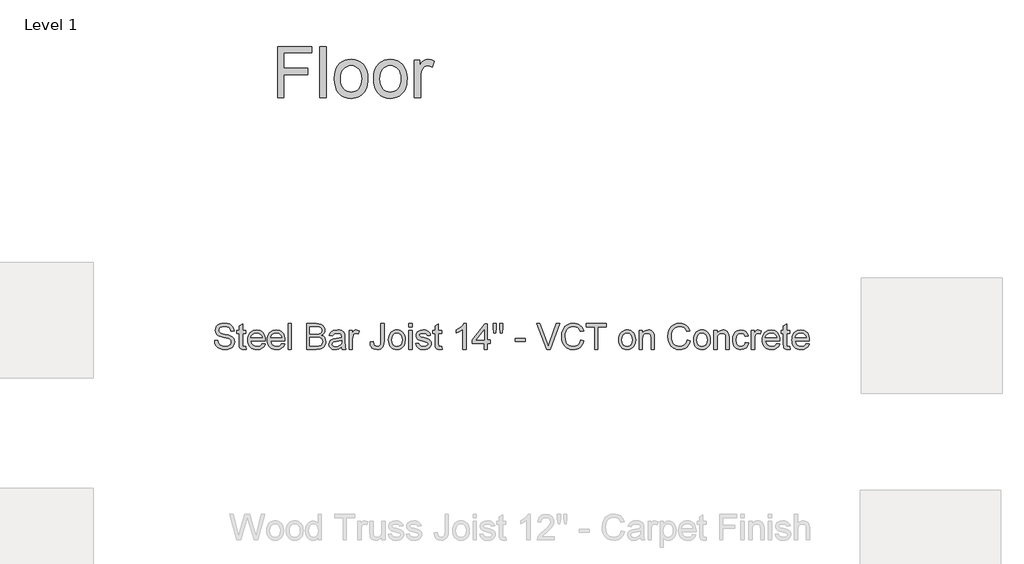
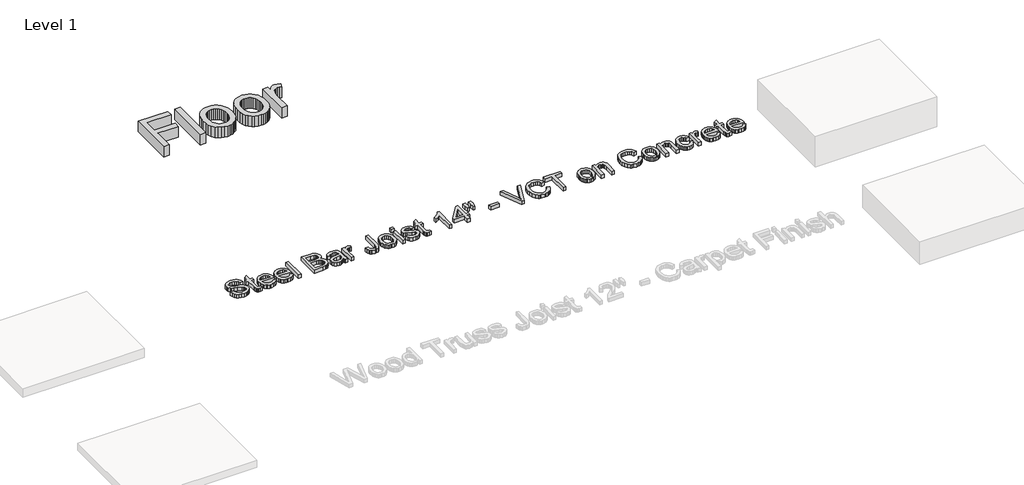
# One storey, part 18 of 42: 2 proxies.
"""IFC4 building model written with IfcOpenShell, lengths in millimetres."""

import ifcopenshell
import ifcopenshell.guid

model = None  # the IFC model being written
_history = None  # IfcOwnerHistory: only IFC2X3 demands one
_inside = {}  # id of a spatial element -> (the spatial element, [elements in it])
_under = {}  # id of a project, library or spatial element -> (it, [spatial elements below it])
_declared = {}  # id of a project -> (the project, [libraries it declares])
_typed = {}  # id of a type object -> (the type object, [elements of that type])
_made_of = {}  # id of a material, layer set ... -> (it, [elements and type objects made of it])


def new_model(schema):
    """Start an empty IFC model of exactly this schema.

    Asked for "IFC4X3", IfcOpenShell would pick the latest addendum, in which some entities
    have other attributes; the version numbers below select the first issue.
    IFC2X3 requires an IfcOwnerHistory on every rooted entity: one is made here for all.
    """
    global model, _history
    if schema == "IFC4X3":
        model = ifcopenshell.file(schema_version=(4, 3, 0, 0))
    else:
        model = ifcopenshell.file(schema=schema)
    _inside.clear()
    _under.clear()
    _declared.clear()
    _typed.clear()
    _made_of.clear()
    _history = None
    if model.schema == "IFC2X3":
        org = make("IfcOrganization", Name="unknown")
        user = make(
            "IfcPersonAndOrganization",
            ThePerson=make("IfcPerson", FamilyName="unknown"),
            TheOrganization=org,
        )
        app = make(
            "IfcApplication",
            ApplicationDeveloper=org,
            Version="unknown",
            ApplicationFullName="unknown",
            ApplicationIdentifier="unknown",
        )
        _history = make(
            "IfcOwnerHistory",
            OwningUser=user,
            OwningApplication=app,
            ChangeAction="ADDED",
            CreationDate=0,
        )
    return model


def make(cls, **values):
    """One entity of the class cls with the attributes given. An attribute that is None is left unset."""
    return model.create_entity(
        cls, **{name: value for name, value in values.items() if value is not None}
    )


def rooted(cls, **values):
    """An entity with a GlobalId (a new one), such as an element, a storey or a relation."""
    return make(cls, GlobalId=ifcopenshell.guid.new(), OwnerHistory=_history, **values)


def si_unit(unit_type, name, prefix=None):
    """IfcSIUnit, for example si_unit("LENGTHUNIT", "METRE", prefix="MILLI")."""
    return make("IfcSIUnit", UnitType=unit_type, Prefix=prefix, Name=name)


def assignment(units):
    """IfcUnitAssignment: the units of a project."""
    return None if units is None else make("IfcUnitAssignment", Units=units)


def point(xyz):
    """IfcCartesianPoint."""
    return None if xyz is None else make("IfcCartesianPoint", Coordinates=xyz)


def direction(xyz):
    """IfcDirection."""
    return None if xyz is None else make("IfcDirection", DirectionRatios=xyz)


def frame(location, z_axis=None, x_axis=None):
    """IfcAxis2Placement3D, a coordinate frame: its origin and axes. An axis left out is left unset."""
    return make(
        "IfcAxis2Placement3D",
        Location=point(location),
        Axis=direction(z_axis),
        RefDirection=direction(x_axis),
    )


def origin():
    """The frame at (0, 0, 0) with its axes left unset."""
    return frame((0.0, 0.0, 0.0))


def origin_with_axes():
    """The frame at (0, 0, 0) with the z axis (0, 0, 1) and the x axis (1, 0, 0) written out."""
    return frame((0.0, 0.0, 0.0), z_axis=(0.0, 0.0, 1.0), x_axis=(1.0, 0.0, 0.0))


def place(relative_to, where):
    """IfcLocalPlacement: puts the frame where relative to a parent placement (None: the world)."""
    return make(
        "IfcLocalPlacement", PlacementRelTo=relative_to, RelativePlacement=where
    )


def context(
    kind, dimensions, precision=None, world=None, true_north=None, identifier=None
):
    """IfcGeometricRepresentationContext, for example the 3D "Model" context."""
    return make(
        "IfcGeometricRepresentationContext",
        ContextIdentifier=identifier,
        ContextType=kind,
        CoordinateSpaceDimension=dimensions,
        Precision=precision,
        WorldCoordinateSystem=world,
        TrueNorth=true_north,
    )


def project(units=None, contexts=None):
    """IfcProject with its units and contexts."""
    return rooted(
        "IfcProject",
        Name="project",
        RepresentationContexts=contexts,
        UnitsInContext=assignment(units),
    )


def spatial(cls, under=None, at=None, **own):
    """A site, building, storey or space (cls), placed at a placement, below another one or the project."""
    s = rooted(cls, ObjectPlacement=at, **own)
    if under is not None:
        _under.setdefault(under.id(), (under, []))[1].append(s)
    return s


def polyline(points):
    """IfcPolyline through the points."""
    return make("IfcPolyline", Points=[point(p) for p in points])


def outline(outer, holes=None, kind="AREA"):
    """IfcArbitraryClosedProfileDef: a profile drawn as a closed curve; with holes, ...WithVoids."""
    if holes is None:
        return make("IfcArbitraryClosedProfileDef", ProfileType=kind, OuterCurve=outer)
    return make(
        "IfcArbitraryProfileDefWithVoids",
        ProfileType=kind,
        OuterCurve=outer,
        InnerCurves=holes,
    )


def extrude(swept, where, along, depth):
    """IfcExtrudedAreaSolid: the profile swept, set in the frame where, extruded along a direction by depth."""
    return make(
        "IfcExtrudedAreaSolid",
        SweptArea=swept,
        Position=where,
        ExtrudedDirection=direction(along),
        Depth=depth,
    )


def shape(context_of_items, identifier, shape_type, items):
    """IfcShapeRepresentation: the items that make up one representation, for example the "Body"."""
    return make(
        "IfcShapeRepresentation",
        ContextOfItems=context_of_items,
        RepresentationIdentifier=identifier,
        RepresentationType=shape_type,
        Items=items,
    )


def made_of(thing, what):
    """Note that an element or type object is made of a material, layer set ...; save() writes the relation."""
    if what is not None:
        _made_of.setdefault(what.id(), (what, []))[1].append(thing)
    return thing


def element(
    cls,
    number,
    at=None,
    inside=None,
    cuts=None,
    type_object=None,
    material=None,
    context=None,
    identifier="Body",
    shape_type=None,
    held_by="IfcProductDefinitionShape",
    body=None,
    shapes=None,
    **own,
):
    """One element of the class cls, such as IfcWall. Its Tag is "e" and its number.

    at: its placement. inside: the storey or other place that contains it. cuts: it is an
    opening in that element (IfcRelVoidsElement). A single representation is given by context,
    identifier, shape_type and body (its items); several are given by shapes. held_by: the class
    of the entity that holds the representations. save() writes the other relations.
    """
    e = rooted(cls, Tag="e%d" % number, ObjectPlacement=at, **own)
    if body is not None:
        shapes = [shape(context, identifier, shape_type, body)]
    if shapes is not None:
        e.Representation = make(held_by, Representations=shapes)
    if inside is not None:
        _inside.setdefault(inside.id(), (inside, []))[1].append(e)
    if cuts is not None:
        rooted(
            "IfcRelVoidsElement", RelatingBuildingElement=cuts, RelatedOpeningElement=e
        )
    if type_object is not None:
        _typed.setdefault(type_object.id(), (type_object, []))[1].append(e)
    return made_of(e, material)


def aggregate(whole, parts):
    """IfcRelAggregates: a whole, such as a stair, and the parts it consists of."""
    return rooted("IfcRelAggregates", RelatingObject=whole, RelatedObjects=parts)


def save(model, path):
    """Write the relations noted so far, then the file.

    IfcRelAggregates (storeys below a building ...), IfcRelContainedInSpatialStructure (elements
    in a storey), IfcRelDefinesByType, IfcRelAssociatesMaterial and IfcRelDeclares: one each for
    every whole, place, type object, material and project.
    """
    for whole, parts in _under.values():
        aggregate(whole, parts)
    for where, things in _inside.values():
        rooted(
            "IfcRelContainedInSpatialStructure",
            RelatedElements=things,
            RelatingStructure=where,
        )
    for kind, things in _typed.values():
        rooted("IfcRelDefinesByType", RelatedObjects=things, RelatingType=kind)
    for what, things in _made_of.values():
        rooted("IfcRelAssociatesMaterial", RelatedObjects=things, RelatingMaterial=what)
    for by, libraries in _declared.values():
        rooted("IfcRelDeclares", RelatingContext=by, RelatedDefinitions=libraries)
    model.write(path)


model = new_model("IFC4")

# Units and contexts
model_context = context("Model", 3, world=origin())
ifc_project = project(units=[si_unit("LENGTHUNIT", "METRE", prefix="MILLI")], contexts=[model_context])

# Site, building, storey
site = spatial("IfcSite", under=ifc_project)
building = spatial("IfcBuilding", under=site)
storey = spatial("IfcBuildingStorey", under=building, Name="Level 1", Elevation=0.0)

# Proxies
placement = place(None, origin())
element("IfcBuildingElementProxy", 1, Name="24\" Arial", ObjectType="24\" Arial", at=placement, inside=storey, context=model_context, shape_type="SweptSolid", body=[
    extrude(outline(polyline([(27657.5158557, -3283.876067), (27657.5158557, -2674.7418789), (28066.7778883, -2674.7418789), (28066.7778883, -2750.8836524), (27733.6576292, -2750.8836524), (27733.6576292, -2931.7203645), (28019.1892799, -2931.7203645), (28019.1892799, -3007.862138), (27733.6576292, -3007.862138), (27733.6576292, -3283.876067), (27657.5158557, -3283.876067)])), origin_with_axes(), (0.0, 0.0, 1.0), 152.4),
    extrude(outline(polyline([(28161.9551052, -3283.876067), (28161.9551052, -2674.7418789), (28238.0968788, -2674.7418789), (28238.0968788, -3283.876067), (28161.9551052, -3283.876067)])), origin_with_axes(), (0.0, 0.0, 1.0), 152.4),
    extrude(outline(polyline([(28333.2740956, -3060.2096073), (28337.3916256, -3002.2760533), (28349.7442156, -2952.3544877), (28370.3318655, -2910.4449104), (28399.1545755, -2876.5473216), (28428.172473, -2854.8814922), (28460.2018372, -2839.4058998), (28495.2426681, -2830.1205444), (28533.2949655, -2827.0254259), (28575.3021366, -2830.7944065), (28613.2847242, -2842.1013483), (28647.2427283, -2860.9462514), (28677.1761489, -2887.3291157), (28701.6071366, -2920.3576548), (28719.0578422, -2959.1395822), (28729.5282655, -3003.6748981), (28733.0184066, -3053.9636024), (28731.4754947, -3094.7206431), (28726.846759, -3130.8861266), (28719.1321994, -3162.4600529), (28708.331816, -3189.4424221), (28694.5803812, -3212.7487572), (28678.0126674, -3233.2945812), (28658.6286746, -3251.0798942), (28636.4284029, -3266.104696), (28612.2762547, -3278.0436741), (28587.0366323, -3286.5715155), (28560.709536, -3291.6882204), (28533.2949655, -3293.3937887), (28490.6743476, -3289.6387501), (28452.3385633, -3278.3736341), (28418.2876127, -3259.598441), (28388.5214958, -3233.3131705), (28364.3507582, -3199.963966), (28347.0859457, -3159.9969706), (28336.7270582, -3113.4121844), (28333.2740956, -3060.2096073)]), holes=[polyline([(28409.4158692, -3060.0608929), (28411.6187012, -3096.993185), (28418.2271974, -3128.9714286), (28429.2413578, -3155.9956238), (28444.6611823, -3178.0657704), (28463.4177862, -3195.2097525), (28484.4422847, -3207.455454), (28507.7346778, -3214.8028749), (28533.2949655, -3217.2520152), (28558.7251282, -3214.7889329), (28581.9245748, -3207.3996861), (28602.8933054, -3195.0842747), (28621.63132, -3177.8426988), (28637.0511445, -3155.5541279), (28648.0653048, -3128.0977315), (28654.673801, -3095.4735097), (28656.8766331, -3057.6814625), (28654.659859, -3021.9202963), (28648.0095369, -2990.7785711), (28636.9256667, -2964.2562871), (28621.4082484, -2942.3534442), (28602.6005239, -2925.2094621), (28581.6457353, -2912.9637606), (28558.5438825, -2905.6163397), (28533.2949655, -2903.1671994), (28507.7346778, -2905.6070451), (28484.4422847, -2912.926582), (28463.4177862, -2925.1258102), (28444.6611823, -2942.2047298), (28429.2413578, -2964.2098139), (28418.2271974, -2991.1875357), (28411.6187012, -3023.1378954), (28409.4158692, -3060.0608929)])]), origin_with_axes(), (0.0, 0.0, 1.0), 152.4),
    extrude(outline(polyline([(28799.6424584, -3060.2096073), (28803.7599884, -3002.2760533), (28816.1125784, -2952.3544877), (28836.7002283, -2910.4449104), (28865.5229383, -2876.5473216), (28894.5408358, -2854.8814922), (28926.5702, -2839.4058998), (28961.6110309, -2830.1205444), (28999.6633283, -2827.0254259), (29041.6704994, -2830.7944065), (29079.653087, -2842.1013483), (29113.6110911, -2860.9462514), (29143.5445117, -2887.3291157), (29167.9754994, -2920.3576548), (29185.426205, -2959.1395822), (29195.8966283, -3003.6748981), (29199.3867694, -3053.9636024), (29197.8438575, -3094.7206431), (29193.2151217, -3130.8861266), (29185.5005622, -3162.4600529), (29174.7001788, -3189.4424221), (29160.948744, -3212.7487572), (29144.3810302, -3233.2945812), (29124.9970374, -3251.0798942), (29102.7967657, -3266.104696), (29078.6446174, -3278.0436741), (29053.4049951, -3286.5715155), (29027.0778988, -3291.6882204), (28999.6633283, -3293.3937887), (28957.0427103, -3289.6387501), (28918.7069261, -3278.3736341), (28884.6559755, -3259.598441), (28854.8898586, -3233.3131705), (28830.719121, -3199.963966), (28813.4543085, -3159.9969706), (28803.0954209, -3113.4121844), (28799.6424584, -3060.2096073)]), holes=[polyline([(28875.784232, -3060.0608929), (28877.987064, -3096.993185), (28884.5955602, -3128.9714286), (28895.6097206, -3155.9956238), (28911.0295451, -3178.0657704), (28929.786149, -3195.2097525), (28950.8106475, -3207.455454), (28974.1030406, -3214.8028749), (28999.6633283, -3217.2520152), (29025.093491, -3214.7889329), (29048.2929376, -3207.3996861), (29069.2616682, -3195.0842747), (29087.9996828, -3177.8426988), (29103.4195073, -3155.5541279), (29114.4336676, -3128.0977315), (29121.0421638, -3095.4735097), (29123.2449959, -3057.6814625), (29121.0282218, -3021.9202963), (29114.3778997, -2990.7785711), (29103.2940295, -2964.2562871), (29087.7766112, -2942.3534442), (29068.9688867, -2925.2094621), (29048.0140981, -2912.9637606), (29024.9122453, -2905.6163397), (28999.6633283, -2903.1671994), (28974.1030406, -2905.6070451), (28950.8106475, -2912.926582), (28929.786149, -2925.1258102), (28911.0295451, -2942.2047298), (28895.6097206, -2964.2098139), (28884.5955602, -2991.1875357), (28877.987064, -3023.1378954), (28875.784232, -3060.0608929)])]), origin_with_axes(), (0.0, 0.0, 1.0), 152.4),
    extrude(outline(polyline([(29285.0462646, -3283.876067), (29285.0462646, -2836.5431476), (29351.6703164, -2836.5431476), (29351.6703164, -2902.7210562), (29376.2825499, -2864.3527407), (29398.9614961, -2841.7481516), (29421.7147995, -2830.7061073), (29446.5501045, -2827.0254259), (29484.4722769, -2832.8996448), (29522.9893069, -2850.5223013), (29497.5591442, -2918.7822116), (29470.790552, -2907.0709525), (29444.0219597, -2903.1671994), (29421.2872456, -2906.9222381), (29400.9691405, -2918.187354), (29384.5547884, -2936.1074393), (29373.5313334, -2959.8273863), (29364.273862, -3002.3597052), (29361.1880381, -3048.7585984), (29361.1880381, -3283.876067), (29285.0462646, -3283.876067)])), origin_with_axes(), (0.0, 0.0, 1.0), 152.4),
])
element("IfcBuildingElementProxy", 2, Name="8\" Arial", ObjectType="8\" Arial", at=placement, inside=storey, context=model_context, shape_type="SweptSolid", body=[
    extrude(outline(polyline([(26907.3095997, -6176.6357974), (26945.3804865, -6176.6357974), (26949.748972, -6197.762537), (26957.6494246, -6214.7438627), (26969.9741306, -6228.2211054), (26987.6153765, -6238.8355958), (27009.1789647, -6245.7229315), (27033.2706977, -6248.0187101), (27054.4810892, -6246.2806105), (27073.0518001, -6241.0663118), (27088.0998386, -6232.8126625), (27098.7422129, -6221.9565112), (27105.0718697, -6209.4923855), (27107.1817552, -6196.4148128), (27105.6016647, -6183.6718475), (27100.8613932, -6172.6576872), (27091.2321357, -6163.2607959), (27074.9850873, -6155.369638), (27019.5517942, -6140.8328053), (26983.1632391, -6131.2128424), (26959.8801406, -6122.0576121), (26940.9283491, -6109.2495843), (26927.4975797, -6093.7275186), (26919.494886, -6075.8260225), (26916.8273214, -6055.8797035), (26920.1269222, -6033.5818379), (26930.0257246, -6012.7897056), (26946.2634783, -5995.1670491), (26968.5799331, -5982.3776106), (26995.3671147, -5974.5979884), (27025.0170484, -5972.0047811), (27057.1393591, -5974.7188189), (27085.246381, -5982.8609324), (27108.3342918, -5996.2638178), (27125.3992694, -6014.7601715), (27136.1996528, -6037.1974568), (27140.4937811, -6062.4231371), (27102.4228944, -6062.4231371), (27095.4333175, -6039.7070123), (27080.8593062, -6023.3112495), (27058.0874135, -6013.3845633), (27026.5041925, -6010.0756678), (26994.1773995, -6013.3473847), (26972.0003643, -6023.1625351), (26959.1737472, -6037.6064214), (26954.8982082, -6054.7643454), (26957.9282641, -6069.3941247), (26967.0184319, -6081.1611517), (26988.5076629, -6091.6826956), (27029.1810517, -6102.4273111), (27071.1556915, -6112.6328369), (27096.5486755, -6121.5371117), (27118.2516835, -6135.3489617), (27133.3926685, -6152.39535), (27142.2876486, -6172.4903835), (27145.252642, -6195.4481692), (27141.8415054, -6218.9171606), (27131.6080957, -6240.9919546), (27114.970672, -6259.9902194), (27092.3474937, -6274.2296233), (27065.1420529, -6283.1246034), (27034.7578417, -6286.0895968), (26997.4584109, -6282.8922372), (26966.7581817, -6273.3001583), (26942.3039573, -6257.2761816), (26923.7425411, -6234.7831283), (26911.8267997, -6207.3824999), (26907.3095997, -6176.6357974)])), origin_with_axes(), (0.0, 0.0, 1.0), 50.8),
    extrude(outline(polyline([(27278.5007456, -6249.5802113), (27283.2596065, -6282.446094), (27254.7807986, -6286.0895968), (27236.5075165, -6284.5095063), (27222.8815595, -6279.7692348), (27213.252302, -6272.4636398), (27206.9691186, -6263.187579), (27203.5115087, -6247.2565488), (27202.3589721, -6219.9860454), (27202.3589721, -6095.735163), (27173.805807, -6095.735163), (27173.805807, -6057.6642763), (27202.3589721, -6057.6642763), (27202.3589721, -6003.3091626), (27240.4298589, -5980.9276451), (27240.4298589, -6057.6642763), (27278.5007456, -6057.6642763), (27278.5007456, -6095.735163), (27240.4298589, -6095.735163), (27240.4298589, -6218.8706874), (27242.4375033, -6238.5009884), (27248.9437584, -6245.4533866), (27261.9190899, -6248.0187101), (27278.5007456, -6249.5802113)])), origin_with_axes(), (0.0, 0.0, 1.0), 50.8),
    extrude(outline(polyline([(27473.1678971, -6214.7066841), (27510.4952118, -6219.465545), (27497.0458531, -6247.5911562), (27475.5845061, -6268.6156547), (27446.5944925, -6281.7211113), (27410.5591341, -6286.0895968), (27386.9367809, -6284.2051065), (27365.8890458, -6278.5516356), (27347.4159287, -6269.1291841), (27331.5174297, -6255.9377519), (27318.7326385, -6239.3444779), (27309.6006448, -6219.7165005), (27304.1214486, -6197.05382), (27302.2950499, -6171.3564361), (27304.1400379, -6144.7876789), (27309.675002, -6121.369808), (27318.8999422, -6101.1028235), (27331.8148585, -6083.9867253), (27347.6715316, -6070.3886522), (27365.7217421, -6060.6757429), (27385.9654899, -6054.8479973), (27408.4027753, -6052.9054154), (27430.1174015, -6054.84335), (27449.7546735, -6060.6571536), (27467.3145912, -6070.3468263), (27482.7971546, -6083.9123681), (27495.435555, -6100.9912877), (27504.4629839, -6121.2210936), (27509.8794413, -6144.6017859), (27511.684927, -6171.1333645), (27511.4618554, -6181.3946582), (27340.3659366, -6181.3946582), (27346.9558435, -6209.8920554), (27362.2641322, -6230.8421967), (27384.3575155, -6243.7245817), (27411.3027061, -6248.0187101), (27431.5650433, -6246.0296549), (27448.6300208, -6240.0624896), (27462.4976388, -6229.745428), (27473.1678971, -6214.7066841)]), holes=[polyline([(27340.3659366, -6143.3237715), (27473.6140403, -6143.3237715), (27468.4648041, -6123.2101487), (27458.3708141, -6108.8220304), (27436.1751897, -6095.4377342), (27408.2540609, -6090.9763022), (27382.591532, -6094.5361532), (27361.3718458, -6105.2157061), (27346.6212361, -6121.8624244), (27340.3659366, -6143.3237715)])]), origin_with_axes(), (0.0, 0.0, 1.0), 50.8),
    extrude(outline(polyline([(27706.3520785, -6214.7066841), (27743.6793932, -6219.465545), (27730.2300345, -6247.5911562), (27708.7686875, -6268.6156547), (27679.7786739, -6281.7211113), (27643.7433155, -6286.0895968), (27620.1209623, -6284.2051065), (27599.0732272, -6278.5516356), (27580.6001101, -6269.1291841), (27564.7016111, -6255.9377519), (27551.9168199, -6239.3444779), (27542.7848262, -6219.7165005), (27537.30563, -6197.05382), (27535.4792313, -6171.3564361), (27537.3242193, -6144.7876789), (27542.8591834, -6121.369808), (27552.0841236, -6101.1028235), (27564.9990399, -6083.9867253), (27580.855713, -6070.3886522), (27598.9059235, -6060.6757429), (27619.1496713, -6054.8479973), (27641.5869567, -6052.9054154), (27663.3015829, -6054.84335), (27682.9388549, -6060.6571536), (27700.4987726, -6070.3468263), (27715.981336, -6083.9123681), (27728.6197364, -6100.9912877), (27737.6471653, -6121.2210936), (27743.0636226, -6144.6017859), (27744.8691084, -6171.1333645), (27744.6460368, -6181.3946582), (27573.550118, -6181.3946582), (27580.1400249, -6209.8920554), (27595.4483136, -6230.8421967), (27617.5416969, -6243.7245817), (27644.4868875, -6248.0187101), (27664.7492247, -6246.0296549), (27681.8142022, -6240.0624896), (27695.6818202, -6229.745428), (27706.3520785, -6214.7066841)]), holes=[polyline([(27573.550118, -6143.3237715), (27706.7982217, -6143.3237715), (27701.6489855, -6123.2101487), (27691.5549955, -6108.8220304), (27669.3593711, -6095.4377342), (27641.4382423, -6090.9763022), (27615.7757134, -6094.5361532), (27594.5560272, -6105.2157061), (27579.8054175, -6121.8624244), (27573.550118, -6143.3237715)])]), origin_with_axes(), (0.0, 0.0, 1.0), 50.8),
    extrude(outline(polyline([(27782.9399952, -6281.330736), (27782.9399952, -5976.7636419), (27821.0108819, -5976.7636419), (27821.0108819, -6281.330736), (27782.9399952, -6281.330736)])), origin_with_axes(), (0.0, 0.0, 1.0), 50.8),
    extrude(outline(polyline([(28001.847594, -6281.330736), (28001.847594, -5976.7636419), (28118.0678987, -5976.7636419), (28150.0322004, -5979.0036526), (28174.9883359, -5985.7236846), (28194.1167258, -5997.0910417), (28208.5977906, -6013.2730275), (28217.7158423, -6032.3084708), (28220.7551929, -6052.2362006), (28218.1991641, -6070.5745452), (28210.5310778, -6087.8161212), (28197.695166, -6102.9013382), (28179.6356609, -6114.7706064), (28201.2085438, -6126.0357223), (28217.1488687, -6143.1750571), (28226.9919031, -6165.0546634), (28230.2729146, -6190.5405939), (28228.0329039, -6211.7788694), (28221.3128719, -6231.4742329), (28211.2839445, -6248.2231924), (28199.1172475, -6260.6222556), (28184.2179234, -6269.6008876), (28165.9911146, -6276.0885533), (28117.1756123, -6281.330736), (28001.847594, -6281.330736)]), holes=[polyline([(28039.9184808, -6100.4940239), (28109.4424635, -6100.4940239), (28150.041495, -6097.222307), (28164.253015, -6091.5804544), (28174.4678355, -6083.1316175), (28180.6301885, -6072.0059214), (28182.6843061, -6058.3334911), (28180.7696082, -6045.0607308), (28175.0255145, -6033.498186), (28165.7122751, -6024.4730808), (28153.0901403, -6018.8126389), (28104.1631022, -6014.8345287), (28039.9184808, -6014.8345287), (28039.9184808, -6100.4940239)]), polyline([(28039.9184808, -6243.2598492), (28117.9935415, -6243.2598492), (28146.2492778, -6241.7727052), (28170.1551178, -6233.4818773), (28185.9932016, -6216.5656142), (28190.6498213, -6204.6126942), (28192.2020278, -6190.9123799), (28190.3802764, -6174.999939), (28184.9150222, -6161.318214), (28175.3694165, -6150.6200718), (28161.3066109, -6143.6583789), (28141.3881758, -6139.8382777), (28114.2756815, -6138.5649106), (28039.9184808, -6138.5649106), (28039.9184808, -6243.2598492)])]), origin_with_axes(), (0.0, 0.0, 1.0), 50.8),
    extrude(outline(polyline([(28420.6273484, -6252.7775709), (28402.4377182, -6268.3739938), (28383.7089982, -6278.5795196), (28364.0136347, -6284.2120775), (28342.9240737, -6286.0895968), (28311.1084864, -6281.5723969), (28287.6394949, -6268.0207971), (28273.1677248, -6247.4424418), (28268.3438014, -6221.8449754), (28270.1655528, -6206.0626596), (28275.630807, -6191.7303091), (28284.0610547, -6179.461371), (28294.7777862, -6169.8692921), (28321.4348427, -6157.3772824), (28354.3750826, -6151.651778), (28393.3010771, -6145.6288447), (28420.4042768, -6138.5649106), (28420.6273484, -6130.0881898), (28418.0062571, -6113.0975694), (28410.1429831, -6101.9811679), (28392.5575051, -6093.7275186), (28368.0568075, -6090.9763022), (28345.3778613, -6092.8073483), (28329.5397775, -6098.3004865), (28318.7393941, -6108.459539), (28311.173549, -6124.2883281), (28273.1026622, -6119.5294673), (28279.7111584, -6098.7094511), (28289.5727822, -6082.3508669), (28303.6077038, -6069.8402679), (28322.7360937, -6060.5642071), (28346.1307279, -6054.8201133), (28372.9643827, -6052.9054154), (28398.7012688, -6054.5970417), (28419.1030258, -6059.6719207), (28434.4856717, -6067.3028284), (28445.1652246, -6076.662541), (28452.247748, -6088.2343804), (28456.8393051, -6102.5016683), (28458.6982351, -6135.8136942), (28458.6982351, -6183.1792311), (28460.6315224, -6249.3199611), (28468.2159568, -6281.330736), (28430.1450701, -6281.330736), (28424.0477796, -6268.0951543), (28420.6273484, -6252.7775709)]), holes=[polyline([(28420.6273484, -6176.6357974), (28359.2083006, -6188.3098779), (28326.4539537, -6194.4815256), (28311.6196922, -6204.5197477), (28306.4146881, -6219.1681162), (28309.2495564, -6230.489), (28317.7541612, -6239.7650608), (28331.7426096, -6245.9552977), (28351.0290085, -6248.0187101), (28371.4772387, -6245.7415208), (28389.5460385, -6238.909953), (28404.194407, -6228.8438469), (28414.3813435, -6216.863043), (28418.8985435, -6204.5197477), (28420.4042768, -6187.4175915), (28420.6273484, -6176.6357974)])]), origin_with_axes(), (0.0, 0.0, 1.0), 50.8),
    extrude(outline(polyline([(28511.0457044, -6281.330736), (28511.0457044, -6057.6642763), (28544.3577304, -6057.6642763), (28544.3577304, -6090.7532306), (28556.6638471, -6071.5690728), (28568.0033202, -6060.2667783), (28579.3799719, -6054.7457561), (28591.7976244, -6052.9054154), (28610.7587106, -6055.8425249), (28630.0172256, -6064.6538531), (28617.3021442, -6098.7838083), (28603.9178481, -6092.9281787), (28590.533552, -6090.9763022), (28579.1661949, -6092.8538215), (28569.0071424, -6098.4863795), (28560.7999664, -6107.4464221), (28555.2882389, -6119.3063957), (28550.6595031, -6140.5725551), (28549.1165912, -6163.7720017), (28549.1165912, -6281.330736), (28511.0457044, -6281.330736)])), origin_with_axes(), (0.0, 0.0, 1.0), 50.8),
    extrude(outline(polyline([(28758.5064684, -6195.8199552), (28796.5773551, -6190.9123799), (28800.5368761, -6218.5918479), (28809.5898653, -6235.8984863), (28823.4203046, -6244.9886541), (28841.712176, -6248.0187101), (28855.7749815, -6246.2991998), (28867.7743748, -6241.140669), (28877.0318463, -6233.0171448), (28882.8688865, -6222.4026544), (28886.9957112, -6184.6663751), (28886.9957112, -5976.7636419), (28925.0665979, -5976.7636419), (28925.0665979, -6183.9971603), (28922.7708194, -6217.8947491), (28915.8834837, -6243.1483134), (28904.0049208, -6261.5981938), (28886.735461, -6275.0847311), (28865.0510423, -6283.3383804), (28839.9276031, -6286.0895968), (28804.7380579, -6280.4105656), (28790.6427211, -6273.3117766), (28778.8803414, -6263.373472), (28769.6600485, -6250.6328304), (28763.190972, -6235.1270304), (28758.5064684, -6195.8199552)])), origin_with_axes(), (0.0, 0.0, 1.0), 50.8),
    extrude(outline(polyline([(28977.4140672, -6169.4975061), (28979.4728322, -6140.5307291), (28985.6491272, -6115.5699463), (28995.9429522, -6094.6151577), (29010.3543071, -6077.6663633), (29024.8632559, -6066.8334486), (29040.877938, -6059.0956524), (29058.3983534, -6054.4529747), (29077.4245022, -6052.9054154), (29098.4280877, -6054.7899057), (29117.4193815, -6060.4433766), (29134.3983836, -6069.8658282), (29149.3650939, -6083.0572603), (29161.5805877, -6099.5715299), (29170.3059405, -6118.9624936), (29175.5411522, -6141.2301515), (29177.2862227, -6166.3745037), (29174.2003989, -6204.8357658), (29164.9429274, -6234.1139135), (29149.7833531, -6256.0399931), (29128.9912209, -6272.4450505), (29104.2953356, -6282.6784602), (29077.4245022, -6286.0895968), (29056.1141932, -6284.2120775), (29036.946301, -6278.5795196), (29019.9208257, -6269.191923), (29005.0377673, -6256.0492877), (28992.9523985, -6239.3746855), (28984.3199922, -6219.3911878), (28979.1405485, -6196.0987947), (28977.4140672, -6169.4975061)]), holes=[polyline([(29015.484954, -6169.4231489), (29019.8906181, -6203.8784168), (29033.1076106, -6228.4255877), (29052.9981617, -6243.1204295), (29077.4245022, -6248.0187101), (29101.7393068, -6243.0925455), (29121.5926794, -6228.3140519), (29134.8096718, -6203.4415682), (29139.215336, -6168.2334337), (29134.7817879, -6134.781988), (29121.4811436, -6110.5694246), (29101.5998871, -6095.8745828), (29077.4245022, -6090.9763022), (29052.9981617, -6095.8559935), (29033.1076106, -6110.4950674), (29019.8906181, -6134.9864703), (29015.484954, -6169.4231489)])]), origin_with_axes(), (0.0, 0.0, 1.0), 50.8),
    extrude(outline(polyline([(29220.1159703, -6281.330736), (29220.1159703, -6057.6642763), (29258.1868571, -6057.6642763), (29258.1868571, -6281.330736), (29220.1159703, -6281.330736)])), origin_with_axes(), (0.0, 0.0, 1.0), 50.8),
    extrude(outline(polyline([(29220.1159703, -6014.8345287), (29220.1159703, -5976.7636419), (29258.1868571, -5976.7636419), (29258.1868571, -6014.8345287), (29220.1159703, -6014.8345287)])), origin_with_axes(), (0.0, 0.0, 1.0), 50.8),
    extrude(outline(polyline([(29301.0166047, -6214.7066841), (29339.0874914, -6209.9478233), (29345.0918354, -6226.2320503), (29356.710148, -6238.2035596), (29374.0167865, -6245.5649224), (29397.086108, -6248.0187101), (29419.87659, -6245.7694047), (29435.9005668, -6239.0214888), (29445.3811098, -6229.2435169), (29448.5412909, -6217.9040438), (29445.3625205, -6208.2004291), (29435.8262096, -6200.8018876), (29396.6399648, -6189.9457363), (29339.310563, -6171.3192575), (29324.8016143, -6161.9595449), (29314.289365, -6149.5697763), (29307.9039404, -6134.9399971), (29305.7754655, -6118.8602524), (29307.4856811, -6104.1096428), (29312.616328, -6090.4929804), (29320.7026736, -6078.549355), (29331.2799854, -6068.8178564), (29355.4832542, -6057.5527405), (29388.2376011, -6052.9054154), (29413.0171382, -6054.7736401), (29434.5621371, -6060.3783141), (29451.8873649, -6069.1710531), (29464.0075886, -6080.6034727), (29472.0381663, -6095.5213861), (29477.0944559, -6114.7706064), (29439.0235692, -6119.5294673), (29434.2182351, -6107.5486633), (29424.709808, -6098.5235581), (29410.4053416, -6092.8631162), (29391.2118891, -6090.9763022), (29369.3508721, -6092.7794643), (29354.7768608, -6098.1889507), (29346.5789794, -6105.9964567), (29343.8463523, -6114.993678), (29348.3821415, -6126.0729009), (29362.5843669, -6134.4752646), (29395.3758924, -6142.5801995), (29451.2553287, -6160.5002848), (29466.015233, -6169.0699522), (29477.2059917, -6180.7998006), (29484.2606312, -6195.7270087), (29486.6121776, -6213.8887549), (29483.8516666, -6232.6639481), (29475.5701333, -6250.3237833), (29462.083596, -6265.4833576), (29443.7080728, -6276.7577681), (29421.5124484, -6283.7566396), (29396.5656076, -6286.0895968), (29358.1787027, -6281.5909862), (29330.1646274, -6268.0951543), (29311.4637914, -6245.7508154), (29301.0166047, -6214.7066841)])), origin_with_axes(), (0.0, 0.0, 1.0), 50.8),
    extrude(outline(polyline([(29610.3425596, -6249.5802113), (29615.1014204, -6282.446094), (29586.6226126, -6286.0895968), (29568.3493305, -6284.5095063), (29554.7233735, -6279.7692348), (29545.094116, -6272.4636398), (29538.8109325, -6263.187579), (29535.3533227, -6247.2565488), (29534.2007861, -6219.9860454), (29534.2007861, -6095.735163), (29505.647621, -6095.735163), (29505.647621, -6057.6642763), (29534.2007861, -6057.6642763), (29534.2007861, -6003.3091626), (29572.2716728, -5980.9276451), (29572.2716728, -6057.6642763), (29610.3425596, -6057.6642763), (29610.3425596, -6095.735163), (29572.2716728, -6095.735163), (29572.2716728, -6218.8706874), (29574.2793173, -6238.5009884), (29580.7855723, -6245.4533866), (29593.7609038, -6248.0187101), (29610.3425596, -6249.5802113)])), origin_with_axes(), (0.0, 0.0, 1.0), 50.8),
    extrude(outline(polyline([(29900.6330711, -6281.330736), (29862.5621844, -6281.330736), (29862.5621844, -6043.9825513), (29826.498942, -6069.6729642), (29786.4204109, -6088.8943006), (29786.4204109, -6052.9054154), (29816.3213002, -6036.6397778), (29842.22549, -6017.2883163), (29862.6458362, -5996.709961), (29876.0951949, -5976.7636419), (29900.6330711, -5976.7636419), (29900.6330711, -6281.330736)])), origin_with_axes(), (0.0, 0.0, 1.0), 50.8),
    extrude(outline(polyline([(30114.7818091, -6281.330736), (30114.7818091, -6209.9478233), (29976.7748446, -6209.9478233), (29976.7748446, -6171.8769365), (30124.2995308, -5981.5225028), (30152.8526959, -5981.5225028), (30152.8526959, -6171.8769365), (30190.9235827, -6171.8769365), (30190.9235827, -6209.9478233), (30152.8526959, -6209.9478233), (30152.8526959, -6281.330736), (30114.7818091, -6281.330736)]), holes=[polyline([(30114.7818091, -6171.8769365), (30114.7818091, -6054.243845), (30023.6198811, -6171.8769365), (30114.7818091, -6171.8769365)])]), origin_with_axes(), (0.0, 0.0, 1.0), 50.8),
    extrude(outline(polyline([(30233.5302587, -6086.2174413), (30224.2356086, -6027.4008956), (30224.2356086, -5976.7636419), (30262.3064953, -5976.7636419), (30262.3064953, -6027.4008956), (30253.9784889, -6086.2174413), (30233.5302587, -6086.2174413)])), origin_with_axes(), (0.0, 0.0, 1.0), 50.8),
    extrude(outline(polyline([(30309.4489606, -6086.2174413), (30300.3773821, -6027.4008956), (30300.3773821, -5976.7636419), (30338.4482689, -5976.7636419), (30338.4482689, -6027.4008956), (30329.5254048, -6086.2174413), (30309.4489606, -6086.2174413)])), origin_with_axes(), (0.0, 0.0, 1.0), 50.8),
    extrude(outline(polyline([(30485.972955, -6190.9123799), (30485.972955, -6152.8414932), (30604.9444762, -6152.8414932), (30604.9444762, -6190.9123799), (30485.972955, -6190.9123799)])), origin_with_axes(), (0.0, 0.0, 1.0), 50.8),
    extrude(outline(polyline([(30861.4768186, -6281.330736), (30740.2745814, -5976.7636419), (30781.0223274, -5976.7636419), (30862.1460334, -6196.1917412), (30878.5789747, -6245.6392796), (30894.7888445, -6196.1917412), (30976.1356221, -5976.7636419), (31016.883368, -5976.7636419), (30900.8117777, -6281.330736), (30861.4768186, -6281.330736)])), origin_with_axes(), (0.0, 0.0, 1.0), 50.8),
    extrude(outline(polyline([(31266.4261336, -6173.0666518), (31304.4970204, -6182.8818022), (31296.9637065, -6206.5575997), (31286.9301317, -6227.2451671), (31274.396296, -6244.9445045), (31259.3621995, -6259.655612), (31242.1670969, -6271.2204803), (31223.1502428, -6279.4811006), (31202.3116373, -6284.4374728), (31179.6512804, -6286.0895968), (31135.4923978, -6281.0890751), (31116.8217694, -6274.8384229), (31100.423683, -6266.0875098), (31073.543555, -6241.6054015), (31053.9504326, -6208.1632505), (31041.9882179, -6168.8468806), (31038.000813, -6126.7421157), (31042.5087183, -6082.3322776), (31056.0324342, -6043.9825513), (31077.8655673, -6012.9105361), (31107.3017241, -5990.333831), (31142.2124298, -5976.5870436), (31180.4692096, -5972.0047811), (31202.2442511, -5973.4872778), (31222.2114831, -5977.9347678), (31240.3709057, -5985.3472513), (31256.7225189, -5995.7247281), (31270.9967778, -6008.7930061), (31282.9241375, -6024.2778932), (31299.7381595, -6062.4974943), (31261.6672727, -6071.5690728), (31248.4688696, -6043.805953), (31230.4372485, -6024.761215), (31207.3493376, -6013.7470546), (31178.9820656, -6010.0756678), (31146.2834866, -6014.1467246), (31119.4219478, -6026.3598948), (31099.0387802, -6045.4325168), (31085.7753145, -6070.0819288), (31078.4976035, -6097.9472897), (31076.0716998, -6126.6677585), (31078.9437467, -6161.8387145), (31087.5598873, -6192.2508095), (31102.2454344, -6216.7422125), (31123.3257008, -6234.1510921), (31148.5978544, -6244.5518056), (31175.8590631, -6248.0187101), (31207.6374718, -6243.2970278), (31234.1179299, -6229.1319811), (31254.1107222, -6205.6722843), (31266.4261336, -6173.0666518)])), origin_with_axes(), (0.0, 0.0, 1.0), 50.8),
    extrude(outline(polyline([(31432.9862632, -6281.330736), (31432.9862632, -6014.8345287), (31333.0501854, -6014.8345287), (31333.0501854, -5976.7636419), (31570.9932277, -5976.7636419), (31570.9932277, -6014.8345287), (31471.0571499, -6014.8345287), (31471.0571499, -6281.330736), (31432.9862632, -6281.330736)])), origin_with_axes(), (0.0, 0.0, 1.0), 50.8),
    extrude(outline(polyline([(31718.5179138, -6169.4975061), (31720.5766788, -6140.5307291), (31726.7529738, -6115.5699463), (31737.0467988, -6094.6151577), (31751.4581538, -6077.6663633), (31765.9671025, -6066.8334486), (31781.9817846, -6059.0956524), (31799.5022001, -6054.4529747), (31818.5283488, -6052.9054154), (31839.5319343, -6054.7899057), (31858.5232281, -6060.4433766), (31875.5022302, -6069.8658282), (31890.4689405, -6083.0572603), (31902.6844343, -6099.5715299), (31911.4097871, -6118.9624936), (31916.6449988, -6141.2301515), (31918.3900693, -6166.3745037), (31915.3042455, -6204.8357658), (31906.046774, -6234.1139135), (31890.8871997, -6256.0399931), (31870.0950675, -6272.4450505), (31845.3991822, -6282.6784602), (31818.5283488, -6286.0895968), (31797.2180398, -6284.2120775), (31778.0501477, -6278.5795196), (31761.0246724, -6269.191923), (31746.1416139, -6256.0492877), (31734.0562451, -6239.3746855), (31725.4238389, -6219.3911878), (31720.2443951, -6196.0987947), (31718.5179138, -6169.4975061)]), holes=[polyline([(31756.5888006, -6169.4231489), (31760.9944647, -6203.8784168), (31774.2114572, -6228.4255877), (31794.1020084, -6243.1204295), (31818.5283488, -6248.0187101), (31842.8431534, -6243.0925455), (31862.696526, -6228.3140519), (31875.9135184, -6203.4415682), (31880.3191826, -6168.2334337), (31875.8856345, -6134.781988), (31862.5849902, -6110.5694246), (31842.7037337, -6095.8745828), (31818.5283488, -6090.9763022), (31794.1020084, -6095.8559935), (31774.2114572, -6110.4950674), (31760.9944647, -6134.9864703), (31756.5888006, -6169.4231489)])]), origin_with_axes(), (0.0, 0.0, 1.0), 50.8),
    extrude(outline(polyline([(31961.2198169, -6281.330736), (31961.2198169, -6057.6642763), (31999.2907037, -6057.6642763), (31999.2907037, -6088.8943006), (32012.5169908, -6073.1491633), (32028.4015478, -6061.9026367), (32046.9443747, -6055.1547207), (32068.1454715, -6052.9054154), (32086.9113701, -6054.7178722), (32104.0971781, -6060.1552425), (32118.4295285, -6068.5390169), (32128.6350543, -6079.1906859), (32140.0488846, -6107.1861719), (32142.056529, -6143.9929863), (32142.056529, -6281.330736), (32103.9856423, -6281.330736), (32103.9856423, -6149.1236331), (32099.5985674, -6115.4398212), (32093.5291609, -6105.4108938), (32084.0950911, -6097.6312716), (32072.0027513, -6092.6400445), (32057.958535, -6090.9763022), (32035.6606695, -6094.7127515), (32016.6531101, -6105.9220995), (32009.0570573, -6115.0726825), (32003.6313053, -6127.5786342), (31999.2907037, -6162.6566437), (31999.2907037, -6281.330736), (31961.2198169, -6281.330736)])), origin_with_axes(), (0.0, 0.0, 1.0), 50.8),
    extrude(outline(polyline([(32532.2831183, -6173.0666518), (32570.3540051, -6182.8818022), (32562.8206912, -6206.5575997), (32552.7871164, -6227.2451671), (32540.2532808, -6244.9445045), (32525.2191842, -6259.655612), (32508.0240816, -6271.2204803), (32489.0072275, -6279.4811006), (32468.168622, -6284.4374728), (32445.5082651, -6286.0895968), (32401.3493825, -6281.0890751), (32382.6787542, -6274.8384229), (32366.2806677, -6266.0875098), (32339.4005397, -6241.6054015), (32319.8074173, -6208.1632505), (32307.8452026, -6168.8468806), (32303.8577978, -6126.7421157), (32308.3657031, -6082.3322776), (32321.8894189, -6043.9825513), (32343.722552, -6012.9105361), (32373.1587088, -5990.333831), (32408.0694145, -5976.5870436), (32446.3261943, -5972.0047811), (32468.1012358, -5973.4872778), (32488.0684678, -5977.9347678), (32506.2278905, -5985.3472513), (32522.5795036, -5995.7247281), (32536.8537625, -6008.7930061), (32548.7811222, -6024.2778932), (32565.5951442, -6062.4974943), (32527.5242575, -6071.5690728), (32514.3258543, -6043.805953), (32496.2942332, -6024.761215), (32473.2063224, -6013.7470546), (32444.8390503, -6010.0756678), (32412.1404713, -6014.1467246), (32385.2789325, -6026.3598948), (32364.8957649, -6045.4325168), (32351.6322992, -6070.0819288), (32344.3545882, -6097.9472897), (32341.9286845, -6126.6677585), (32344.8007314, -6161.8387145), (32353.416872, -6192.2508095), (32368.1024192, -6216.7422125), (32389.1826856, -6234.1510921), (32414.4548392, -6244.5518056), (32441.7160479, -6248.0187101), (32473.4944565, -6243.2970278), (32499.9749146, -6229.1319811), (32519.9677069, -6205.6722843), (32532.2831183, -6173.0666518)])), origin_with_axes(), (0.0, 0.0, 1.0), 50.8),
    extrude(outline(polyline([(32608.4248918, -6169.4975061), (32610.4836568, -6140.5307291), (32616.6599518, -6115.5699463), (32626.9537768, -6094.6151577), (32641.3651317, -6077.6663633), (32655.8740805, -6066.8334486), (32671.8887626, -6059.0956524), (32689.409178, -6054.4529747), (32708.4353268, -6052.9054154), (32729.4389123, -6054.7899057), (32748.4302061, -6060.4433766), (32765.4092081, -6069.8658282), (32780.3759184, -6083.0572603), (32792.5914123, -6099.5715299), (32801.3167651, -6118.9624936), (32806.5519768, -6141.2301515), (32808.2970473, -6166.3745037), (32805.2112235, -6204.8357658), (32795.953752, -6234.1139135), (32780.7941777, -6256.0399931), (32760.0020455, -6272.4450505), (32735.3061602, -6282.6784602), (32708.4353268, -6286.0895968), (32687.1250178, -6284.2120775), (32667.9571256, -6278.5795196), (32650.9316503, -6269.191923), (32636.0485919, -6256.0492877), (32623.9632231, -6239.3746855), (32615.3308168, -6219.3911878), (32610.1513731, -6196.0987947), (32608.4248918, -6169.4975061)]), holes=[polyline([(32646.4957786, -6169.4231489), (32650.9014427, -6203.8784168), (32664.1184352, -6228.4255877), (32684.0089863, -6243.1204295), (32708.4353268, -6248.0187101), (32732.7501314, -6243.0925455), (32752.603504, -6228.3140519), (32765.8204964, -6203.4415682), (32770.2261606, -6168.2334337), (32765.7926125, -6134.781988), (32752.4919682, -6110.5694246), (32732.6107116, -6095.8745828), (32708.4353268, -6090.9763022), (32684.0089863, -6095.8559935), (32664.1184352, -6110.4950674), (32650.9014427, -6134.9864703), (32646.4957786, -6169.4231489)])]), origin_with_axes(), (0.0, 0.0, 1.0), 50.8),
    extrude(outline(polyline([(32851.1267949, -6281.330736), (32851.1267949, -6057.6642763), (32889.1976817, -6057.6642763), (32889.1976817, -6088.8943006), (32902.4239687, -6073.1491633), (32918.3085257, -6061.9026367), (32936.8513527, -6055.1547207), (32958.0524495, -6052.9054154), (32976.818348, -6054.7178722), (32994.0041561, -6060.1552425), (33008.3365065, -6068.5390169), (33018.5420323, -6079.1906859), (33029.9558626, -6107.1861719), (33031.963507, -6143.9929863), (33031.963507, -6281.330736), (32993.8926203, -6281.330736), (32993.8926203, -6149.1236331), (32989.5055454, -6115.4398212), (32983.4361389, -6105.4108938), (32974.0020691, -6097.6312716), (32961.9097293, -6092.6400445), (32947.865513, -6090.9763022), (32925.5676475, -6094.7127515), (32906.560088, -6105.9220995), (32898.9640353, -6115.0726825), (32893.5382833, -6127.5786342), (32889.1976817, -6162.6566437), (32889.1976817, -6281.330736), (32851.1267949, -6281.330736)])), origin_with_axes(), (0.0, 0.0, 1.0), 50.8),
    extrude(outline(polyline([(33227.0768017, -6200.4301016), (33265.1476884, -6205.1889625), (33254.533198, -6239.0493727), (33234.5868789, -6264.6375444), (33207.1862505, -6280.7265837), (33174.208832, -6286.0895968), (33152.856697, -6284.2190485), (33133.7120415, -6278.6074035), (33116.7748654, -6269.2546619), (33102.0451687, -6256.1608235), (33090.1224563, -6239.5721968), (33081.6062331, -6219.7350898), (33076.4964993, -6196.6495027), (33074.7932546, -6170.3154353), (33077.7024801, -6136.4364358), (33086.4301565, -6107.0746361), (33101.1157037, -6083.3639838), (33121.8985413, -6066.438426), (33146.7617302, -6056.2886681), (33173.6883316, -6052.9054154), (33205.8571155, -6057.5527405), (33231.5754123, -6071.4947156), (33250.0252927, -6093.9877688), (33260.3888276, -6124.2883281), (33222.3179408, -6129.0471889), (33215.4120158, -6112.4376492), (33204.6581056, -6100.5312025), (33190.651068, -6093.3650273), (33173.9857604, -6090.9763022), (33149.3828216, -6095.6793951), (33129.8547617, -6109.788674), (33117.1117965, -6134.0663), (33112.8641414, -6169.2744345), (33117.01885, -6204.9565962), (33129.4829757, -6229.3178741), (33148.6578389, -6243.3435011), (33172.9447595, -6248.0187101), (33192.6587124, -6245.1001899), (33208.8221089, -6236.3446296), (33220.5798412, -6221.5289573), (33227.0768017, -6200.4301016)])), origin_with_axes(), (0.0, 0.0, 1.0), 50.8),
    extrude(outline(polyline([(33298.4597143, -6281.330736), (33298.4597143, -6057.6642763), (33331.7717402, -6057.6642763), (33331.7717402, -6090.7532306), (33344.077857, -6071.5690728), (33355.4173301, -6060.2667783), (33366.7939818, -6054.7457561), (33379.2116343, -6052.9054154), (33398.1727205, -6055.8425249), (33417.4312354, -6064.6538531), (33404.7161541, -6098.7838083), (33391.331858, -6092.9281787), (33377.9475619, -6090.9763022), (33366.5802048, -6092.8538215), (33356.4211523, -6098.4863795), (33348.2139762, -6107.4464221), (33342.7022487, -6119.3063957), (33338.073513, -6140.5725551), (33336.5306011, -6163.7720017), (33336.5306011, -6281.330736), (33298.4597143, -6281.330736)])), origin_with_axes(), (0.0, 0.0, 1.0), 50.8),
    extrude(outline(polyline([(33597.8218043, -6214.7066841), (33635.1491191, -6219.465545), (33621.6997604, -6247.5911562), (33600.2384134, -6268.6156547), (33571.2483997, -6281.7211113), (33535.2130414, -6286.0895968), (33511.5906882, -6284.2051065), (33490.542953, -6278.5516356), (33472.069836, -6269.1291841), (33456.171337, -6255.9377519), (33443.3865458, -6239.3444779), (33434.2545521, -6219.7165005), (33428.7753559, -6197.05382), (33426.9489571, -6171.3564361), (33428.7939452, -6144.7876789), (33434.3289093, -6121.369808), (33443.5538495, -6101.1028235), (33456.4687658, -6083.9867253), (33472.3254389, -6070.3886522), (33490.3756493, -6060.6757429), (33510.6193972, -6054.8479973), (33533.0566825, -6052.9054154), (33554.7713088, -6054.84335), (33574.4085808, -6060.6571536), (33591.9684985, -6070.3468263), (33607.4510618, -6083.9123681), (33620.0894623, -6100.9912877), (33629.1168912, -6121.2210936), (33634.5333485, -6144.6017859), (33636.3388343, -6171.1333645), (33636.1157627, -6181.3946582), (33465.0198439, -6181.3946582), (33471.6097508, -6209.8920554), (33486.9180395, -6230.8421967), (33509.0114228, -6243.7245817), (33535.9566134, -6248.0187101), (33556.2189506, -6246.0296549), (33573.2839281, -6240.0624896), (33587.151546, -6229.745428), (33597.8218043, -6214.7066841)]), holes=[polyline([(33465.0198439, -6143.3237715), (33598.2679476, -6143.3237715), (33593.1187114, -6123.2101487), (33583.0247214, -6108.8220304), (33560.829097, -6095.4377342), (33532.9079681, -6090.9763022), (33507.2454392, -6094.5361532), (33486.0257531, -6105.2157061), (33471.2751434, -6121.8624244), (33465.0198439, -6143.3237715)])]), origin_with_axes(), (0.0, 0.0, 1.0), 50.8),
    extrude(outline(polyline([(33755.3103554, -6249.5802113), (33760.0692163, -6282.446094), (33731.5904084, -6286.0895968), (33713.3171263, -6284.5095063), (33699.6911693, -6279.7692348), (33690.0619118, -6272.4636398), (33683.7787284, -6263.187579), (33680.3211185, -6247.2565488), (33679.1685819, -6219.9860454), (33679.1685819, -6095.735163), (33650.6154168, -6095.735163), (33650.6154168, -6057.6642763), (33679.1685819, -6057.6642763), (33679.1685819, -6003.3091626), (33717.2394687, -5980.9276451), (33717.2394687, -6057.6642763), (33755.3103554, -6057.6642763), (33755.3103554, -6095.735163), (33717.2394687, -6095.735163), (33717.2394687, -6218.8706874), (33719.2471131, -6238.5009884), (33725.7533682, -6245.4533866), (33738.7286997, -6248.0187101), (33755.3103554, -6249.5802113)])), origin_with_axes(), (0.0, 0.0, 1.0), 50.8),
    extrude(outline(polyline([(33949.9775069, -6214.7066841), (33987.3048216, -6219.465545), (33973.8554629, -6247.5911562), (33952.3941159, -6268.6156547), (33923.4041023, -6281.7211113), (33887.3687439, -6286.0895968), (33863.7463907, -6284.2051065), (33842.6986556, -6278.5516356), (33824.2255385, -6269.1291841), (33808.3270395, -6255.9377519), (33795.5422483, -6239.3444779), (33786.4102546, -6219.7165005), (33780.9310584, -6197.05382), (33779.1046597, -6171.3564361), (33780.9496477, -6144.7876789), (33786.4846118, -6121.369808), (33795.709552, -6101.1028235), (33808.6244683, -6083.9867253), (33824.4811414, -6070.3886522), (33842.5313519, -6060.6757429), (33862.7750997, -6054.8479973), (33885.2123851, -6052.9054154), (33906.9270113, -6054.84335), (33926.5642833, -6060.6571536), (33944.124201, -6070.3468263), (33959.6067644, -6083.9123681), (33972.2451648, -6100.9912877), (33981.2725937, -6121.2210936), (33986.689051, -6144.6017859), (33988.4945368, -6171.1333645), (33988.2714652, -6181.3946582), (33817.1755464, -6181.3946582), (33823.7654533, -6209.8920554), (33839.073742, -6230.8421967), (33861.1671253, -6243.7245817), (33888.1123159, -6248.0187101), (33908.3746531, -6246.0296549), (33925.4396306, -6240.0624896), (33939.3072486, -6229.745428), (33949.9775069, -6214.7066841)]), holes=[polyline([(33817.1755464, -6143.3237715), (33950.4236501, -6143.3237715), (33945.2744139, -6123.2101487), (33935.1804239, -6108.8220304), (33912.9847995, -6095.4377342), (33885.0636707, -6090.9763022), (33859.4011418, -6094.5361532), (33838.1814556, -6105.2157061), (33823.4308459, -6121.8624244), (33817.1755464, -6143.3237715)])]), origin_with_axes(), (0.0, 0.0, 1.0), 50.8),
])

save(model, "model.ifc")

# Revit data of these elements
# Element 1 (IfcBuildingElementProxy, "24\" Arial")
#   Phase Created = New Construction
# Element 2 (IfcBuildingElementProxy, "8\" Arial")
#   Phase Created = New Construction
